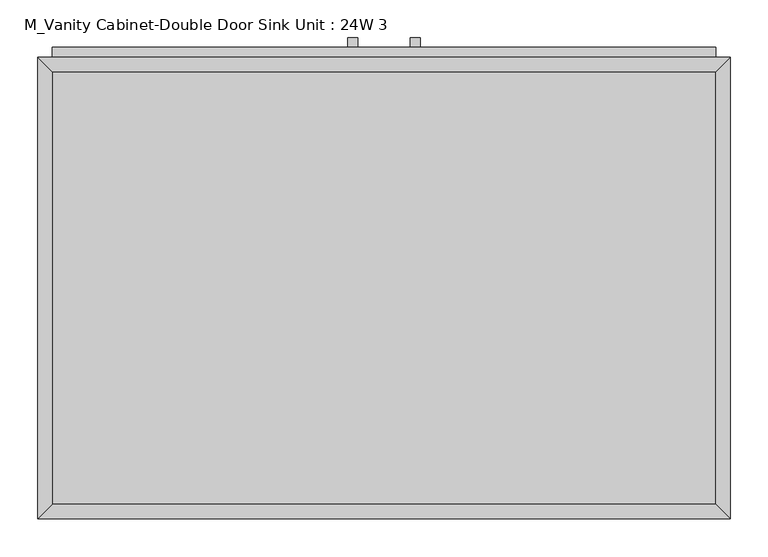
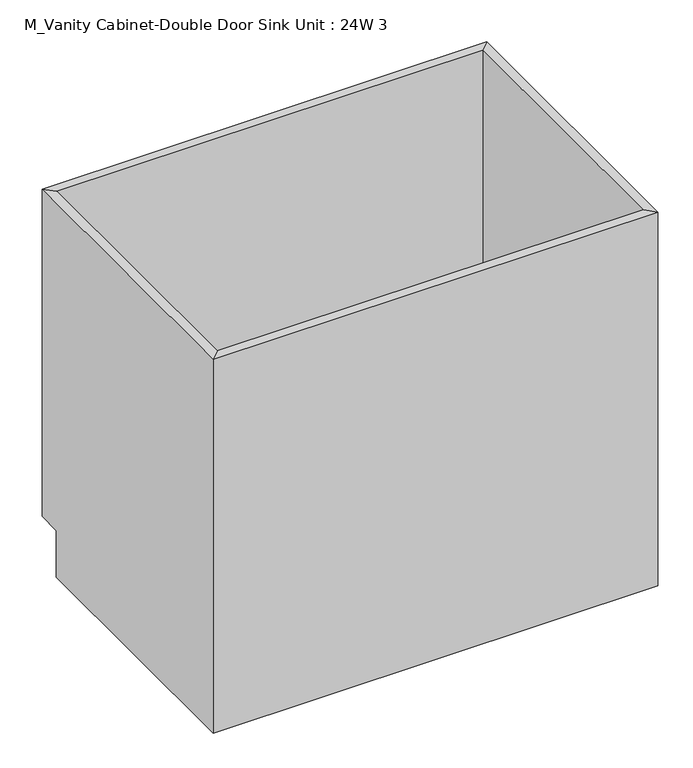
"""IFC4 building model written with IfcOpenShell, lengths in millimetres: furniture geometry, M_Vanity Cabinet-Double Door Sink Unit : 24W 3."""

from ifc_helpers import new_model, si_unit, frame, origin, place, context, project, spatial, polyline, outline, extrude, faceted_brep, source, transform, mapped, element, save


def m_vanity_cabinet_double_door_sink_unit_24w_3_5d6bdcb6(model_context):
    return source(origin(), model_context, "Body", "SolidModel", [
        faceted_brep([(456.8877049, 590.55, 812.8), (-419.4122951, 590.55, 812.8), (-419.4122951, 590.55, 101.6), (456.8877049, 590.55, 101.6), (475.9377049, 609.6, 812.8), (-438.4622951, 609.6, 812.8), (475.9377049, 609.6, 101.6), (-438.4622951, 609.6, 101.6), (-419.4122951, 19.05, 812.8), (-419.4122951, 19.05, 101.6), (-419.4122951, 558.8, 101.6), (-438.4622951, 0.0, 812.8), (-438.4622951, 558.8, 101.6), (-438.4622951, 558.8, 0.0), (-438.4622951, 0.0, 0.0), (456.8877049, 19.05, 812.8), (456.8877049, 19.05, 101.6), (475.9377049, 0.0, 812.8), (475.9377049, 0.0, 0.0), (456.8877049, 558.8, 101.6), (475.9377049, 558.8, 0.0), (475.9377049, 558.8, 101.6)], [[[0, 1, 2, 3]], [[0, 4, 5, 1]], [[4, 6, 7, 5]], [[2, 7, 6, 3]], [[1, 8, 9, 10, 2]], [[5, 11, 8, 1]], [[7, 12, 13, 14, 11, 5]], [[2, 10, 12, 7]], [[8, 15, 16, 9]], [[11, 17, 15, 8]], [[14, 18, 17, 11]], [[3, 19, 16, 15, 0]], [[0, 15, 17, 4]], [[4, 17, 18, 20, 21, 6]], [[6, 21, 19, 3]], [[10, 9, 16, 19]], [[18, 14, 13, 20]], [[13, 12, 10, 19, 21, 20]]]),
        extrude(outline(polyline([(-16.1872951, 635.0), (-16.1872951, 622.3), (-28.8872951, 622.3), (-28.8872951, 635.0), (-16.1872951, 635.0)])), frame((0.0, 0.0, 510.269895), z_axis=(0.0, 0.0, 1.0), x_axis=(1.0, 0.0, 0.0)), (0.0, 0.0, 1.0), 124.730105),
        extrude(outline(polyline([(66.3627049, 635.0), (66.3627049, 622.3), (53.6627049, 622.3), (53.6627049, 635.0), (66.3627049, 635.0)])), frame((0.0, 0.0, 510.269895), z_axis=(0.0, 0.0, 1.0), x_axis=(1.0, 0.0, 0.0)), (0.0, 0.0, 1.0), 124.730105),
        extrude(outline(polyline([(9.2127049, 622.3), (9.2127049, 609.6), (-419.4122951, 609.6), (-419.4122951, 622.3), (9.2127049, 622.3)])), frame((0.0, 0.0, 120.65), z_axis=(0.0, 0.0, 1.0), x_axis=(1.0, 0.0, 0.0)), (0.0, 0.0, 1.0), 552.45),
        extrude(outline(polyline([(456.8877049, 622.3), (456.8877049, 609.6), (28.2627049, 609.6), (28.2627049, 622.3), (456.8877049, 622.3)])), frame((0.0, 0.0, 120.65), z_axis=(0.0, 0.0, 1.0), x_axis=(1.0, 0.0, 0.0)), (0.0, 0.0, 1.0), 552.45),
        extrude(outline(polyline([(456.8877049, 622.3), (456.8877049, 609.6), (-419.4122951, 609.6), (-419.4122951, 622.3), (456.8877049, 622.3)])), frame((0.0, 0.0, 692.15), z_axis=(0.0, 0.0, 1.0), x_axis=(1.0, 0.0, 0.0)), (0.0, 0.0, 1.0), 101.6),
        extrude(outline(polyline([(456.8877049, 19.05), (-419.4122951, 19.05), (-419.4122951, 590.55), (456.8877049, 590.55), (456.8877049, 19.05)])), frame((0.0, 0.0, 101.6), z_axis=(0.0, 0.0, 1.0), x_axis=(1.0, 0.0, 0.0)), (0.0, 0.0, 1.0), 19.05),
    ])


if __name__ == "__main__":
    model = new_model("IFC4")
    model_context = context("Model", 3, world=origin())
    ifc_project = project(units=[si_unit("LENGTHUNIT", "METRE", prefix="MILLI")], contexts=[model_context])
    site = spatial("IfcSite", under=ifc_project)
    building = spatial("IfcBuilding", under=site)
    placement = place(None, origin())
    m_vanity_cabinet_double_door_sink_unit_24w_3_shape = m_vanity_cabinet_double_door_sink_unit_24w_3_5d6bdcb6(model_context)
    element("IfcFurniture", 1, ObjectType="M_Vanity Cabinet-Double Door Sink Unit : 24W 3", at=placement, inside=building, context=model_context, shape_type="MappedRepresentation", body=[
        mapped(m_vanity_cabinet_double_door_sink_unit_24w_3_shape, transform((0.0, 0.0, 0.0), x_axis=(1.0, 0.0, 0.0), y_axis=(0.0, 1.0, 0.0), z_axis=(0.0, 0.0, 1.0))),
    ])
    save(model, "model.ifc")

# Revit data of these elements
# Type "M_Vanity Cabinet-Double Door Sink Unit : 24W 3"
#   Depth = 2' - 0"
#   Height = 2' - 8"
#   Plinth Depth = 0' - 2"
#   Plinth Height = 0' - 4"
#   Width = 3' - 0"
#   Cabinet Material = none
#   Door/Drawer Material = none
#   Handle Material = Cabinets - Handles
# Element 1 (IfcFurniture, "M_Vanity Cabinet-Double Door Sink Unit : 24W 3")
#   Materials on its faces: "MAX HEIGHT OF  COUNTERTOP 34\"", "Cabinets - Handles"
# Materials
#   "Cabinets - Handles": class "Metal", colour RGB 57 57 57, transparency 0
#   "MAX HEIGHT OF  COUNTERTOP 34\"": class "Generic", colour RGB 181 181 181, transparency 0, Cost = 0
